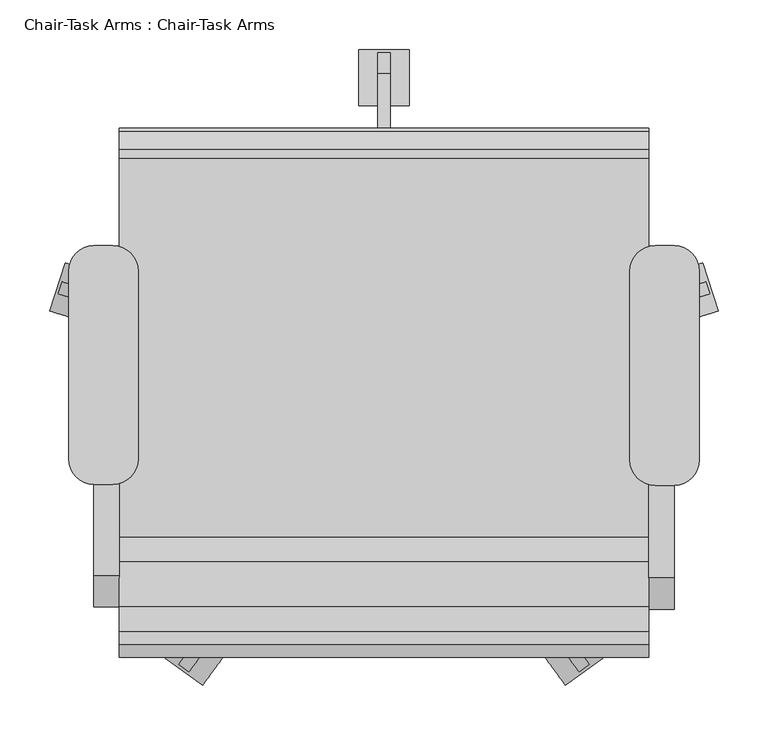
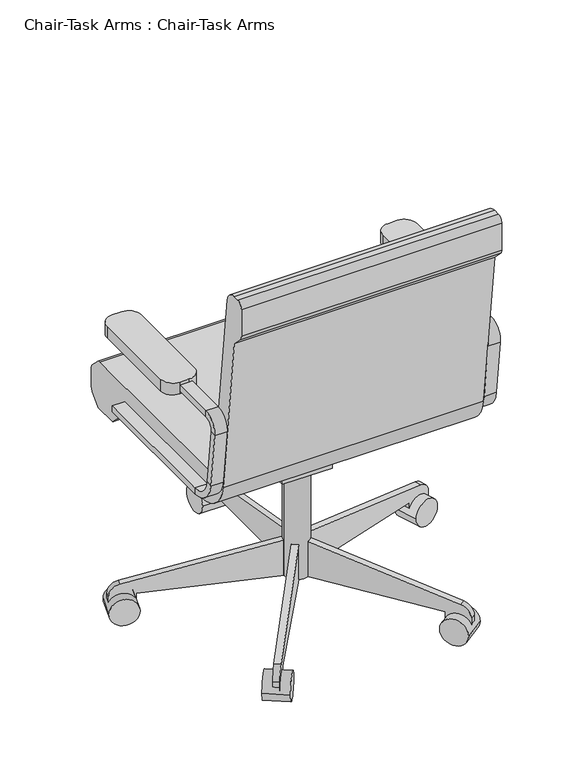
"""IFC4 building model written with IfcOpenShell, lengths in millimetres: furniture geometry, Chair-Task Arms : Chair-Task Arms."""

import ifcopenshell
import ifcopenshell.guid

model = None  # the IFC model being written
_history = None  # IfcOwnerHistory: only IFC2X3 demands one
_inside = {}  # id of a spatial element -> (the spatial element, [elements in it])
_under = {}  # id of a project, library or spatial element -> (it, [spatial elements below it])
_declared = {}  # id of a project -> (the project, [libraries it declares])
_typed = {}  # id of a type object -> (the type object, [elements of that type])
_made_of = {}  # id of a material, layer set ... -> (it, [elements and type objects made of it])


def new_model(schema):
    """Start an empty IFC model of exactly this schema.

    Asked for "IFC4X3", IfcOpenShell would pick the latest addendum, in which some entities
    have other attributes; the version numbers below select the first issue.
    IFC2X3 requires an IfcOwnerHistory on every rooted entity: one is made here for all.
    """
    global model, _history
    if schema == "IFC4X3":
        model = ifcopenshell.file(schema_version=(4, 3, 0, 0))
    else:
        model = ifcopenshell.file(schema=schema)
    _inside.clear()
    _under.clear()
    _declared.clear()
    _typed.clear()
    _made_of.clear()
    _history = None
    if model.schema == "IFC2X3":
        org = make("IfcOrganization", Name="unknown")
        user = make(
            "IfcPersonAndOrganization",
            ThePerson=make("IfcPerson", FamilyName="unknown"),
            TheOrganization=org,
        )
        app = make(
            "IfcApplication",
            ApplicationDeveloper=org,
            Version="unknown",
            ApplicationFullName="unknown",
            ApplicationIdentifier="unknown",
        )
        _history = make(
            "IfcOwnerHistory",
            OwningUser=user,
            OwningApplication=app,
            ChangeAction="ADDED",
            CreationDate=0,
        )
    return model


def make(cls, **values):
    """One entity of the class cls with the attributes given. An attribute that is None is left unset."""
    return model.create_entity(
        cls, **{name: value for name, value in values.items() if value is not None}
    )


def rooted(cls, **values):
    """An entity with a GlobalId (a new one), such as an element, a storey or a relation."""
    return make(cls, GlobalId=ifcopenshell.guid.new(), OwnerHistory=_history, **values)


def si_unit(unit_type, name, prefix=None):
    """IfcSIUnit, for example si_unit("LENGTHUNIT", "METRE", prefix="MILLI")."""
    return make("IfcSIUnit", UnitType=unit_type, Prefix=prefix, Name=name)


def assignment(units):
    """IfcUnitAssignment: the units of a project."""
    return None if units is None else make("IfcUnitAssignment", Units=units)


def point(xyz):
    """IfcCartesianPoint."""
    return None if xyz is None else make("IfcCartesianPoint", Coordinates=xyz)


def direction(xyz):
    """IfcDirection."""
    return None if xyz is None else make("IfcDirection", DirectionRatios=xyz)


def frame(location, z_axis=None, x_axis=None):
    """IfcAxis2Placement3D, a coordinate frame: its origin and axes. An axis left out is left unset."""
    return make(
        "IfcAxis2Placement3D",
        Location=point(location),
        Axis=direction(z_axis),
        RefDirection=direction(x_axis),
    )


def frame_2d(location, x_axis=None):
    """IfcAxis2Placement2D, a coordinate frame in the plane: its origin and x axis."""
    return make(
        "IfcAxis2Placement2D", Location=point(location), RefDirection=direction(x_axis)
    )


def origin():
    """The frame at (0, 0, 0) with its axes left unset."""
    return frame((0.0, 0.0, 0.0))


def place(relative_to, where):
    """IfcLocalPlacement: puts the frame where relative to a parent placement (None: the world)."""
    return make(
        "IfcLocalPlacement", PlacementRelTo=relative_to, RelativePlacement=where
    )


def context(
    kind, dimensions, precision=None, world=None, true_north=None, identifier=None
):
    """IfcGeometricRepresentationContext, for example the 3D "Model" context."""
    return make(
        "IfcGeometricRepresentationContext",
        ContextIdentifier=identifier,
        ContextType=kind,
        CoordinateSpaceDimension=dimensions,
        Precision=precision,
        WorldCoordinateSystem=world,
        TrueNorth=true_north,
    )


def project(units=None, contexts=None):
    """IfcProject with its units and contexts."""
    return rooted(
        "IfcProject",
        Name="project",
        RepresentationContexts=contexts,
        UnitsInContext=assignment(units),
    )


def spatial(cls, under=None, at=None, **own):
    """A site, building, storey or space (cls), placed at a placement, below another one or the project."""
    s = rooted(cls, ObjectPlacement=at, **own)
    if under is not None:
        _under.setdefault(under.id(), (under, []))[1].append(s)
    return s


def polyline(points):
    """IfcPolyline through the points."""
    return make("IfcPolyline", Points=[point(p) for p in points])


def circle_curve(where, radius):
    """IfcCircle in the frame where."""
    return make("IfcCircle", Position=where, Radius=radius)


def trimmed(basis, trim1, trim2, sense, master):
    """IfcTrimmedCurve: the piece of a basis curve between two trims."""
    return make(
        "IfcTrimmedCurve",
        BasisCurve=basis,
        Trim1=trim1,
        Trim2=trim2,
        SenseAgreement=sense,
        MasterRepresentation=master,
    )


def segment(curve, same_sense, transition):
    """IfcCompositeCurveSegment."""
    return make(
        "IfcCompositeCurveSegment",
        Transition=transition,
        SameSense=same_sense,
        ParentCurve=curve,
    )


def composite_curve(segments, self_intersect=None):
    """IfcCompositeCurve: segments joined end to end."""
    return make("IfcCompositeCurve", Segments=segments, SelfIntersect=self_intersect)


def outline(outer, holes=None, kind="AREA"):
    """IfcArbitraryClosedProfileDef: a profile drawn as a closed curve; with holes, ...WithVoids."""
    if holes is None:
        return make("IfcArbitraryClosedProfileDef", ProfileType=kind, OuterCurve=outer)
    return make(
        "IfcArbitraryProfileDefWithVoids",
        ProfileType=kind,
        OuterCurve=outer,
        InnerCurves=holes,
    )


def extrude(swept, where, along, depth):
    """IfcExtrudedAreaSolid: the profile swept, set in the frame where, extruded along a direction by depth."""
    return make(
        "IfcExtrudedAreaSolid",
        SweptArea=swept,
        Position=where,
        ExtrudedDirection=direction(along),
        Depth=depth,
    )


def shape(context_of_items, identifier, shape_type, items):
    """IfcShapeRepresentation: the items that make up one representation, for example the "Body"."""
    return make(
        "IfcShapeRepresentation",
        ContextOfItems=context_of_items,
        RepresentationIdentifier=identifier,
        RepresentationType=shape_type,
        Items=items,
    )


def source(mapping_origin, context_of_items, identifier, shape_type, items):
    """IfcRepresentationMap: a shape defined once, which mapped items show again and again."""
    return make(
        "IfcRepresentationMap",
        MappingOrigin=mapping_origin,
        MappedRepresentation=shape(context_of_items, identifier, shape_type, items),
    )


def transform(
    local_origin,
    x_axis=None,
    y_axis=None,
    z_axis=None,
    scale=None,
    scale2=None,
    scale3=None,
    uniform=True,
):
    """IfcCartesianTransformationOperator3D, or its non-uniform kind. x_axis, y_axis, z_axis: its Axis1, 2, 3."""
    if uniform:
        return make(
            "IfcCartesianTransformationOperator3D",
            Axis1=direction(x_axis),
            Axis2=direction(y_axis),
            LocalOrigin=point(local_origin),
            Scale=scale,
            Axis3=direction(z_axis),
        )
    return make(
        "IfcCartesianTransformationOperator3DnonUniform",
        Axis1=direction(x_axis),
        Axis2=direction(y_axis),
        LocalOrigin=point(local_origin),
        Scale=scale,
        Axis3=direction(z_axis),
        Scale2=scale2,
        Scale3=scale3,
    )


def mapped(mapping_source, mapping_target):
    """IfcMappedItem: shows the shape of a source again, moved by a transform."""
    return make(
        "IfcMappedItem", MappingSource=mapping_source, MappingTarget=mapping_target
    )


def made_of(thing, what):
    """Note that an element or type object is made of a material, layer set ...; save() writes the relation."""
    if what is not None:
        _made_of.setdefault(what.id(), (what, []))[1].append(thing)
    return thing


def element(
    cls,
    number,
    at=None,
    inside=None,
    cuts=None,
    type_object=None,
    material=None,
    context=None,
    identifier="Body",
    shape_type=None,
    held_by="IfcProductDefinitionShape",
    body=None,
    shapes=None,
    **own,
):
    """One element of the class cls, such as IfcWall. Its Tag is "e" and its number.

    at: its placement. inside: the storey or other place that contains it. cuts: it is an
    opening in that element (IfcRelVoidsElement). A single representation is given by context,
    identifier, shape_type and body (its items); several are given by shapes. held_by: the class
    of the entity that holds the representations. save() writes the other relations.
    """
    e = rooted(cls, Tag="e%d" % number, ObjectPlacement=at, **own)
    if body is not None:
        shapes = [shape(context, identifier, shape_type, body)]
    if shapes is not None:
        e.Representation = make(held_by, Representations=shapes)
    if inside is not None:
        _inside.setdefault(inside.id(), (inside, []))[1].append(e)
    if cuts is not None:
        rooted(
            "IfcRelVoidsElement", RelatingBuildingElement=cuts, RelatedOpeningElement=e
        )
    if type_object is not None:
        _typed.setdefault(type_object.id(), (type_object, []))[1].append(e)
    return made_of(e, material)


def aggregate(whole, parts):
    """IfcRelAggregates: a whole, such as a stair, and the parts it consists of."""
    return rooted("IfcRelAggregates", RelatingObject=whole, RelatedObjects=parts)


def save(model, path):
    """Write the relations noted so far, then the file.

    IfcRelAggregates (storeys below a building ...), IfcRelContainedInSpatialStructure (elements
    in a storey), IfcRelDefinesByType, IfcRelAssociatesMaterial and IfcRelDeclares: one each for
    every whole, place, type object, material and project.
    """
    for whole, parts in _under.values():
        aggregate(whole, parts)
    for where, things in _inside.values():
        rooted(
            "IfcRelContainedInSpatialStructure",
            RelatedElements=things,
            RelatingStructure=where,
        )
    for kind, things in _typed.values():
        rooted("IfcRelDefinesByType", RelatedObjects=things, RelatingType=kind)
    for what, things in _made_of.values():
        rooted("IfcRelAssociatesMaterial", RelatedObjects=things, RelatingMaterial=what)
    for by, libraries in _declared.values():
        rooted("IfcRelDeclares", RelatingContext=by, RelatedDefinitions=libraries)
    model.write(path)


def plane_surface(at):
    """IfcPlane: the flat surface through the origin of the frame at, square to its z axis."""
    return make("IfcPlane", Position=at)


def cylinder_surface(at, radius):
    """IfcCylindricalSurface: all points at the distance radius from the z axis of the frame at."""
    return make("IfcCylindricalSurface", Position=at, Radius=radius)


def revolved_surface(curve, axis_point, axis_direction):
    """IfcSurfaceOfRevolution: the curve turned about the line through axis_point along axis_direction."""
    return make(
        "IfcSurfaceOfRevolution",
        SweptCurve=make("IfcArbitraryOpenProfileDef", ProfileType="CURVE", Curve=curve),
        AxisPosition=make("IfcAxis1Placement", Location=point(axis_point), Axis=direction(axis_direction)),
    )


def advanced_brep(points, edges, surfaces, faces):
    """IfcAdvancedBrep: a solid bounded by faces that lie on surfaces and meet in shared edges.

    An edge is (start, end): straight between two places in points (the first is 0);
    or (start, end, curve); or (start, end, curve, False) where it runs against its curve.
    A face is (place in surfaces, loops), or (place, loops, False) where it looks against
    its surface's normal. A loop lists edges by number (the first is 1), with a minus sign
    where the edge is run from its end to its start. The first loop is the outer one.
    """
    corners = [point(p) for p in points]
    vertices = [make("IfcVertexPoint", VertexGeometry=c) for c in corners]
    made = []
    for start, end, *more in edges:
        made.append(
            make(
                "IfcEdgeCurve",
                EdgeStart=vertices[start],
                EdgeEnd=vertices[end],
                EdgeGeometry=more[0] if more else make("IfcPolyline", Points=[corners[start], corners[end]]),
                SameSense=more[1] if len(more) > 1 else True,
            )
        )
    hull = []
    for where, loops, *sense in faces:
        bounds = []
        for j, loop in enumerate(loops):
            ring = [make("IfcOrientedEdge", EdgeElement=made[abs(k) - 1], Orientation=k > 0) for k in loop]
            bounds.append(
                make(
                    "IfcFaceOuterBound" if j == 0 else "IfcFaceBound",
                    Bound=make("IfcEdgeLoop", EdgeList=ring),
                    Orientation=True,
                )
            )
        hull.append(make("IfcAdvancedFace", Bounds=bounds, FaceSurface=surfaces[where], SameSense=sense[0] if sense else True))
    return make("IfcAdvancedBrep", Outer=make("IfcClosedShell", CfsFaces=hull))


def chair_task_arms_chair_task_arms_fa5a08ef(model_context):
    return source(origin(), model_context, "Body", "SolidModel", [
        extrude(outline(composite_curve([segment(polyline([(433.0908197, -74.2028048), (414.0408197, -74.2028048)]), True, "CONTINUOUS"), segment(trimmed(circle_curve(frame_2d((414.0408197, -48.8028048)), 25.4), [point((414.0408197, -74.2028048))], [point((388.6408197, -48.8028048))], False, "CARTESIAN"), True, "CONTINUOUS"), segment(polyline([(388.6408197, -48.8028048), (388.6408197, 141.6319091)]), True, "CONTINUOUS"), segment(trimmed(circle_curve(frame_2d((414.0408197, 141.6319091)), 25.4), [point((388.6408197, 141.6319091))], [point((414.0408197, 167.0319091))], False, "CARTESIAN"), True, "CONTINUOUS"), segment(polyline([(414.0408197, 167.0319091), (433.0908197, 167.0319091)]), True, "CONTINUOUS"), segment(trimmed(circle_curve(frame_2d((433.0908197, 141.6319091)), 25.4), [point((433.0908197, 167.0319091))], [point((458.4908197, 141.6319091))], False, "CARTESIAN"), True, "CONTINUOUS"), segment(polyline([(458.4908197, 141.6319091), (458.4908197, -48.8028048)]), True, "CONTINUOUS"), segment(trimmed(circle_curve(frame_2d((433.0908197, -48.8028048)), 25.4), [point((458.4908197, -48.8028048))], [point((433.0908197, -74.2028048))], False, "CARTESIAN"), True, "CONTINUOUS")], self_intersect=False)), frame((0.0, 0.0, 596.9), z_axis=(0.0, 0.0, 1.0), x_axis=(1.0, 0.0, 0.0)), (0.0, 0.0, 1.0), 25.4),
        extrude(outline(composite_curve([segment(polyline([(-132.0591803, -73.1575984), (-151.1091803, -73.1575984)]), True, "CONTINUOUS"), segment(trimmed(circle_curve(frame_2d((-151.1091803, -47.7575984)), 25.4), [point((-151.1091803, -73.1575984))], [point((-176.5091803, -47.7575984))], False, "CARTESIAN"), True, "CONTINUOUS"), segment(polyline([(-176.5091803, -47.7575984), (-176.5091803, 141.6319091)]), True, "CONTINUOUS"), segment(trimmed(circle_curve(frame_2d((-151.1091803, 141.6319091)), 25.4), [point((-176.5091803, 141.6319091))], [point((-151.1091803, 167.0319091))], False, "CARTESIAN"), True, "CONTINUOUS"), segment(polyline([(-151.1091803, 167.0319091), (-132.0591803, 167.0319091)]), True, "CONTINUOUS"), segment(trimmed(circle_curve(frame_2d((-132.0591803, 141.6319091)), 25.4), [point((-132.0591803, 167.0319091))], [point((-106.6591803, 141.6319091))], False, "CARTESIAN"), True, "CONTINUOUS"), segment(polyline([(-106.6591803, 141.6319091), (-106.6591803, -47.7575984)]), True, "CONTINUOUS"), segment(trimmed(circle_curve(frame_2d((-132.0591803, -47.7575984)), 25.4), [point((-106.6591803, -47.7575984))], [point((-132.0591803, -73.1575984))], False, "CARTESIAN"), True, "CONTINUOUS")], self_intersect=False)), frame((0.0, 0.0, 596.9), z_axis=(0.0, 0.0, 1.0), x_axis=(1.0, 0.0, 0.0)), (0.0, 0.0, 1.0), 25.4),
        advanced_brep(
        [(-151.1091803, 167.0319091, 412.75), (-151.1091803, 167.0319091, 425.45), (-125.7091803, 167.0319091, 425.45), (-125.7091803, 167.0319091, 412.75), (-151.1091803, -126.2388651, 412.75), (-151.1091803, -126.2388651, 425.45), (-125.7091803, -126.2388651, 425.45), (-125.7091803, -126.2388651, 412.75), (-151.1091803, -170.3844094, 464.7064065), (-151.1091803, -182.9974221, 463.2225227), (-125.7091803, -170.3844094, 464.7064065), (-125.7091803, -182.9974221, 463.2225227), (-151.1091803, -196.7936301, 580.4902904), (-151.1091803, -184.1806174, 581.9741742), (-125.7091803, -184.1806174, 581.9741742), (-125.7091803, -196.7936301, 580.4902904), (-151.1091803, -165.2610984, 603.25), (-151.1091803, -165.2610984, 615.95), (-125.7091803, -165.2610984, 603.25), (-125.7091803, -165.2610984, 615.95), (-151.1091803, 18.9459016, 615.95), (-125.7091803, 18.9459016, 615.95), (-125.7091803, 18.9459016, 603.25), (-151.1091803, 18.9459016, 603.25)],
        [
            (0, 1),
            (1, 2),
            (2, 3),
            (3, 0),
            (0, 4),
            (4, 5),
            (5, 1),
            (5, 6),
            (6, 2),
            (6, 7),
            (7, 3),
            (7, 4),
            (8, 5, circle_curve(frame((-151.1091803, -126.2388651, 469.9), z_axis=(1.0, 0.0, 0.0), x_axis=(0.0, 0.0, -1.0)), 44.45)),
            (4, 9, circle_curve(frame((-151.1091803, -126.2388651, 469.9), z_axis=(-1.0, 0.0, 0.0), x_axis=(0.0, 0.0, -1.0)), 57.15)),
            (9, 8),
            (10, 6, circle_curve(frame((-125.7091803, -126.2388651, 469.9), z_axis=(1.0, 0.0, 0.0), x_axis=(0.0, 0.0, -1.0)), 44.45)),
            (8, 10),
            (11, 7, circle_curve(frame((-125.7091803, -126.2388651, 469.9), z_axis=(1.0, 0.0, 0.0), x_axis=(0.0, 0.0, -1.0)), 57.15)),
            (10, 11),
            (11, 9),
            (9, 12),
            (12, 13),
            (13, 8),
            (13, 14),
            (14, 10),
            (14, 15),
            (15, 11),
            (15, 12),
            (16, 13, circle_curve(frame((-151.1091803, -165.2610984, 584.2), z_axis=(1.0, 0.0, 0.0), x_axis=(0.0, -0.9931506043228768, -0.11684124756739202)), 19.05)),
            (12, 17, circle_curve(frame((-151.1091803, -165.2610984, 584.2), z_axis=(-1.0, 0.0, 0.0), x_axis=(0.0, -0.9931506043228768, -0.11684124756739202)), 31.75)),
            (17, 16),
            (18, 14, circle_curve(frame((-125.7091803, -165.2610984, 584.2), z_axis=(1.0, 0.0, 0.0), x_axis=(0.0, -0.9931506043228768, -0.11684124756739202)), 19.05)),
            (16, 18),
            (19, 15, circle_curve(frame((-125.7091803, -165.2610984, 584.2), z_axis=(1.0, 0.0, 0.0), x_axis=(0.0, -0.9931506043228768, -0.11684124756739202)), 31.75)),
            (18, 19),
            (19, 17),
            (20, 21),
            (21, 22),
            (22, 23),
            (23, 20),
            (17, 20),
            (23, 16),
            (22, 18),
            (21, 19),
        ],
        [
            plane_surface(frame((-152.608212, 167.0319091, 419.1), z_axis=(0.0, 1.0, 0.0), x_axis=(0.0, 0.0, -1.0))),
            plane_surface(frame((-151.1091803, 167.0319091, 412.75), z_axis=(-1.0, 0.0, 0.0), x_axis=(0.0, -1.0, 0.0))),
            plane_surface(frame((-151.1091803, 167.0319091, 425.45), z_axis=(0.0, 0.0, 1.0), x_axis=(0.0, -1.0, 0.0))),
            plane_surface(frame((-125.7091803, 167.0319091, 425.45), z_axis=(1.0, 0.0, 0.0), x_axis=(0.0, -1.0, 0.0))),
            plane_surface(frame((-125.7091803, 167.0319091, 412.75), z_axis=(0.0, 0.0, -1.0), x_axis=(0.0, -1.0, 0.0))),
            plane_surface(frame((-151.1091803, -126.2388651, 469.9), z_axis=(-1.0, 0.0, 0.0), x_axis=(0.0, 0.0, -1.0))),
            revolved_surface(polyline([(-151.1091803, -126.2388651, 425.45), (-125.7091803, -126.2388651, 425.45)]), (-138.4091803, -126.2388651, 469.9), (-1.0, 0.0, 0.0)),
            plane_surface(frame((-125.7091803, -126.2388651, 469.9), z_axis=(1.0, 0.0, 0.0), x_axis=(0.0, 0.0, -1.0))),
            cylinder_surface(frame((-138.4091803, -126.2388651, 469.9), z_axis=(-1.0, 0.0, 0.0), x_axis=(0.0, 0.0, -1.0)), 57.15),
            plane_surface(frame((-151.1091803, -182.9974221, 463.2225227), z_axis=(-1.0, 0.0, 0.0), x_axis=(0.0, -0.1168412475673856, 0.9931506043228776))),
            plane_surface(frame((-151.1091803, -170.3844094, 464.7064065), z_axis=(0.0, 0.9931506043228776, 0.1168412475673856), x_axis=(0.0, -0.1168412475673856, 0.9931506043228776))),
            plane_surface(frame((-125.7091803, -170.3844094, 464.7064065), z_axis=(1.0, 0.0, 0.0), x_axis=(0.0, -0.1168412475673856, 0.9931506043228776))),
            plane_surface(frame((-125.7091803, -182.9974221, 463.2225227), z_axis=(0.0, -0.9931506043228776, -0.1168412475673856), x_axis=(0.0, -0.1168412475673856, 0.9931506043228776))),
            plane_surface(frame((-151.1091803, -165.2610984, 584.2), z_axis=(-1.0, 0.0, 0.0), x_axis=(0.0, -0.9931506043228768, -0.11684124756739202))),
            revolved_surface(polyline([(-151.1091803, -184.1806174123508, 581.9741742338413), (-125.7091803, -184.1806174123508, 581.9741742338413)]), (-138.4091803, -165.2610984, 584.2), (-1.0, 0.0, 0.0)),
            plane_surface(frame((-125.7091803, -165.2610984, 584.2), z_axis=(1.0, 0.0, 0.0), x_axis=(0.0, -0.9931506043228768, -0.11684124756739202))),
            cylinder_surface(frame((-138.4091803, -165.2610984, 584.2), z_axis=(-1.0, 0.0, 0.0), x_axis=(0.0, -0.9931506043228768, -0.11684124756739202)), 31.75),
            plane_surface(frame((-152.608212, 18.9459016, 609.6), z_axis=(0.0, 1.0, 0.0), x_axis=(0.0, 0.0, 1.0))),
            plane_surface(frame((-151.1091803, -165.2610984, 615.95), z_axis=(-1.0, 0.0, 0.0), x_axis=(0.0, 1.0, 0.0))),
            plane_surface(frame((-151.1091803, -165.2610984, 603.25), z_axis=(0.0, 0.0, -1.0), x_axis=(0.0, 1.0, 0.0))),
            plane_surface(frame((-125.7091803, -165.2610984, 603.25), z_axis=(1.0, 0.0, 0.0), x_axis=(0.0, 1.0, 0.0))),
            plane_surface(frame((-125.7091803, -165.2610984, 615.95), z_axis=(0.0, 0.0, 1.0), x_axis=(0.0, 1.0, 0.0))),
        ],
        [
            (0, [[1, 2, 3, 4]]),
            (1, [[-1, 5, 6, 7]]),
            (2, [[-2, -7, 8, 9]]),
            (3, [[-3, -9, 10, 11]]),
            (4, [[-4, -11, 12, -5]]),
            (5, [[13, -6, 14, 15]]),
            (6, [[16, -8, -13, 17]]),
            (7, [[18, -10, -16, 19]]),
            (8, [[-14, -12, -18, 20]]),
            (9, [[-15, 21, 22, 23]]),
            (10, [[-17, -23, 24, 25]]),
            (11, [[-19, -25, 26, 27]]),
            (12, [[-20, -27, 28, -21]]),
            (13, [[29, -22, 30, 31]]),
            (14, [[32, -24, -29, 33]]),
            (15, [[34, -26, -32, 35]]),
            (16, [[-30, -28, -34, 36]]),
            (17, [[37, 38, 39, 40]]),
            (18, [[-31, 41, -40, 42]]),
            (19, [[-33, -42, -39, 43]]),
            (20, [[-35, -43, -38, 44]]),
            (21, [[-36, -44, -37, -41]]),
        ],
    ),
        advanced_brep(
        [(433.0908197, 167.0319091, 425.45), (433.0908197, 167.0319091, 412.75), (407.6908197, 167.0319091, 412.75), (407.6908197, 167.0319091, 425.45), (433.0908197, -128.329278, 425.45), (433.0908197, -128.329278, 412.75), (407.6908197, -128.329278, 412.75), (407.6908197, -128.329278, 425.45), (433.0908197, -185.0878351, 463.2225227), (433.0908197, -172.4748224, 464.7064065), (407.6908197, -185.0878351, 463.2225227), (407.6908197, -172.4748224, 464.7064065), (433.0908197, -186.2710303, 581.9741742), (433.0908197, -198.884043, 580.4902904), (407.6908197, -198.884043, 580.4902904), (407.6908197, -186.2710303, 581.9741742), (433.0908197, -167.3515113, 615.95), (433.0908197, -167.3515113, 603.25), (407.6908197, -167.3515113, 615.95), (407.6908197, -167.3515113, 603.25), (433.0908197, 18.9459016, 603.25), (407.6908197, 18.9459016, 603.25), (407.6908197, 18.9459016, 615.95), (433.0908197, 18.9459016, 615.95)],
        [
            (0, 1),
            (1, 2),
            (2, 3),
            (3, 0),
            (0, 4),
            (4, 5),
            (5, 1),
            (5, 6),
            (6, 2),
            (6, 7),
            (7, 3),
            (7, 4),
            (8, 5, circle_curve(frame((433.0908197, -128.329278, 469.9), z_axis=(1.0, 0.0, 0.0), x_axis=(0.0, 0.0, -1.0)), 57.15)),
            (4, 9, circle_curve(frame((433.0908197, -128.329278, 469.9), z_axis=(-1.0, 0.0, 0.0), x_axis=(0.0, 0.0, -1.0)), 44.45)),
            (9, 8),
            (10, 6, circle_curve(frame((407.6908197, -128.329278, 469.9), z_axis=(1.0, 0.0, 0.0), x_axis=(0.0, 0.0, -1.0)), 57.15)),
            (8, 10),
            (11, 7, circle_curve(frame((407.6908197, -128.329278, 469.9), z_axis=(1.0, 0.0, 0.0), x_axis=(0.0, 0.0, -1.0)), 44.45)),
            (10, 11),
            (11, 9),
            (9, 12),
            (12, 13),
            (13, 8),
            (13, 14),
            (14, 10),
            (14, 15),
            (15, 11),
            (15, 12),
            (16, 13, circle_curve(frame((433.0908197, -167.3515113, 584.2), z_axis=(1.0, 0.0, 0.0), x_axis=(0.0, -0.9931506043228767, -0.1168412475673929)), 31.75)),
            (12, 17, circle_curve(frame((433.0908197, -167.3515113, 584.2), z_axis=(-1.0, 0.0, 0.0), x_axis=(0.0, -0.9931506043228767, -0.1168412475673929)), 19.05)),
            (17, 16),
            (18, 14, circle_curve(frame((407.6908197, -167.3515113, 584.2), z_axis=(1.0, 0.0, 0.0), x_axis=(0.0, -0.9931506043228767, -0.1168412475673929)), 31.75)),
            (16, 18),
            (19, 15, circle_curve(frame((407.6908197, -167.3515113, 584.2), z_axis=(1.0, 0.0, 0.0), x_axis=(0.0, -0.9931506043228767, -0.1168412475673929)), 19.05)),
            (18, 19),
            (19, 17),
            (20, 21),
            (21, 22),
            (22, 23),
            (23, 20),
            (17, 20),
            (23, 16),
            (22, 18),
            (21, 19),
        ],
        [
            plane_surface(frame((406.191788, 167.0319091, 419.1), z_axis=(0.0, 1.0, 0.0), x_axis=(0.0, 0.0, -1.0))),
            plane_surface(frame((433.0908197, 167.0319091, 425.45), z_axis=(1.0, 0.0, 0.0), x_axis=(0.0, -1.0, 0.0))),
            plane_surface(frame((433.0908197, 167.0319091, 412.75), z_axis=(0.0, 0.0, -1.0), x_axis=(0.0, -1.0, 0.0))),
            plane_surface(frame((407.6908197, 167.0319091, 412.75), z_axis=(-1.0, 0.0, 0.0), x_axis=(0.0, -1.0, 0.0))),
            plane_surface(frame((407.6908197, 167.0319091, 425.45), z_axis=(0.0, 0.0, 1.0), x_axis=(0.0, -1.0, 0.0))),
            plane_surface(frame((433.0908197, -128.329278, 469.9), z_axis=(1.0, 0.0, 0.0), x_axis=(0.0, 0.0, -1.0))),
            cylinder_surface(frame((420.3908197, -128.329278, 469.9), z_axis=(-1.0, 0.0, 0.0), x_axis=(0.0, 0.0, -1.0)), 57.15),
            plane_surface(frame((407.6908197, -128.329278, 469.9), z_axis=(-1.0, 0.0, 0.0), x_axis=(0.0, 0.0, -1.0))),
            revolved_surface(polyline([(407.6908197, -128.329278, 425.45), (433.0908197, -128.329278, 425.45)]), (420.3908197, -128.329278, 469.9), (-1.0, 0.0, 0.0)),
            plane_surface(frame((433.0908197, -172.4748224, 464.7064065), z_axis=(1.0, 0.0, 0.0), x_axis=(0.0, -0.11684124756738626, 0.9931506043228775))),
            plane_surface(frame((433.0908197, -185.0878351, 463.2225227), z_axis=(0.0, -0.9931506043228775, -0.11684124756738655), x_axis=(0.0, -0.11684124756738655, 0.9931506043228775))),
            plane_surface(frame((407.6908197, -185.0878351, 463.2225227), z_axis=(-1.0, 0.0, 0.0), x_axis=(0.0, -0.11684124756738626, 0.9931506043228775))),
            plane_surface(frame((407.6908197, -172.4748224, 464.7064065), z_axis=(0.0, 0.9931506043228775, 0.11684124756738626), x_axis=(0.0, -0.11684124756738626, 0.9931506043228775))),
            plane_surface(frame((433.0908197, -167.3515113, 584.2), z_axis=(1.0, 0.0, 0.0), x_axis=(0.0, -0.9931506043228767, -0.1168412475673929))),
            cylinder_surface(frame((420.3908197, -167.3515113, 584.2), z_axis=(-1.0, 0.0, 0.0), x_axis=(0.0, -0.9931506043228767, -0.1168412475673929)), 31.75),
            plane_surface(frame((407.6908197, -167.3515113, 584.2), z_axis=(-1.0, 0.0, 0.0), x_axis=(0.0, -0.9931506043228767, -0.1168412475673929))),
            revolved_surface(polyline([(407.6908197, -186.2710303123508, 581.9741742338412), (433.0908197, -186.2710303123508, 581.9741742338412)]), (420.3908197, -167.3515113, 584.2), (-1.0, 0.0, 0.0)),
            plane_surface(frame((406.191788, 18.9459016, 609.6), z_axis=(0.0, 1.0, 0.0), x_axis=(0.0, 0.0, 1.0))),
            plane_surface(frame((433.0908197, -167.3515113, 603.25), z_axis=(1.0, 0.0, 0.0), x_axis=(0.0, 1.0, 0.0))),
            plane_surface(frame((433.0908197, -167.3515113, 615.95), z_axis=(0.0, 0.0, 1.0), x_axis=(0.0, 1.0, 0.0))),
            plane_surface(frame((407.6908197, -167.3515113, 615.95), z_axis=(-1.0, 0.0, 0.0), x_axis=(0.0, 1.0, 0.0))),
            plane_surface(frame((407.6908197, -167.3515113, 603.25), z_axis=(0.0, 0.0, -1.0), x_axis=(0.0, 1.0, 0.0))),
        ],
        [
            (0, [[1, 2, 3, 4]]),
            (1, [[-1, 5, 6, 7]]),
            (2, [[-2, -7, 8, 9]]),
            (3, [[-3, -9, 10, 11]]),
            (4, [[-4, -11, 12, -5]]),
            (5, [[13, -6, 14, 15]]),
            (6, [[16, -8, -13, 17]]),
            (7, [[18, -10, -16, 19]]),
            (8, [[-14, -12, -18, 20]]),
            (9, [[-15, 21, 22, 23]]),
            (10, [[-17, -23, 24, 25]]),
            (11, [[-19, -25, 26, 27]]),
            (12, [[-20, -27, 28, -21]]),
            (13, [[29, -22, 30, 31]]),
            (14, [[32, -24, -29, 33]]),
            (15, [[34, -26, -32, 35]]),
            (16, [[-30, -28, -34, 36]]),
            (17, [[37, 38, 39, 40]]),
            (18, [[-31, 41, -40, 42]]),
            (19, [[-33, -42, -39, 43]]),
            (20, [[-35, -43, -38, 44]]),
            (21, [[-36, -44, -37, -41]]),
        ],
    ),
        extrude(outline(composite_curve([segment(trimmed(circle_curve(frame_2d((140.9908197, 18.9459016)), 25.4), [point((115.5908197, 18.9459016))], [point((166.3908197, 18.9459016))], False, "CARTESIAN"), True, "CONTINUOUS"), segment(trimmed(circle_curve(frame_2d((140.9908197, 18.9459016)), 25.4), [point((166.3908197, 18.9459016))], [point((115.5908197, 18.9459016))], False, "CARTESIAN"), True, "CONTINUOUS")], self_intersect=False)), frame((0.0, 0.0, 53.5835944), z_axis=(0.0, 0.0, 1.0), x_axis=(1.0, 0.0, 0.0)), (0.0, 0.0, 1.0), 330.5914056),
        extrude(outline(composite_curve([segment(trimmed(circle_curve(frame_2d((0.0, -28.2002727)), 28.2002727), [point((0.0, -56.4005455))], [point((0.0, 0.0))], False, "CARTESIAN"), True, "CONTINUOUS"), segment(trimmed(circle_curve(frame_2d((0.0, -28.2002727)), 28.2002727), [point((0.0, 0.0))], [point((0.0, -56.4005455))], False, "CARTESIAN"), True, "CONTINUOUS")], self_intersect=False)), frame((477.6203484, 101.6163254, 28.1835944), z_axis=(-0.3090169943749423, 0.9510565162951553, 0.0), x_axis=(0.0, 0.0, 1.0)), (0.0, 0.0, 1.0), 50.8),
        extrude(outline(composite_curve([segment(polyline([(-25.4, 0.0), (0.0, 0.0), (0.0, -50.8), (-24.303053, -50.8)]), True, "CONTINUOUS"), segment(trimmed(circle_curve(frame_2d((-24.303053, -25.4)), 25.4), [point((-24.303053, -50.8))], [point((-49.3171699, -29.8106637))], False, "CARTESIAN"), True, "CONTINUOUS"), segment(polyline([(-49.3171699, -29.8106637), (-101.6, 266.7), (-101.6, 292.1), (-25.4, 292.1), (-25.4, 0.0)]), True, "CONTINUOUS")], self_intersect=False)), frame((420.756686, 103.1705568, 28.1835944), z_axis=(-0.3090169943749423, 0.9510565162951553, 0.0), x_axis=(0.0, 0.0, -1.0)), (0.0, 0.0, 1.0), 12.7),
        extrude(outline(composite_curve([segment(trimmed(circle_curve(frame_2d((0.0, -28.2002727)), 28.2002727), [point((0.0, -56.4005455))], [point((0.0, 0.0))], False, "CARTESIAN"), True, "CONTINUOUS"), segment(trimmed(circle_curve(frame_2d((0.0, -28.2002727)), 28.2002727), [point((0.0, 0.0))], [point((0.0, -56.4005455))], False, "CARTESIAN"), True, "CONTINUOUS")], self_intersect=False)), frame((323.63931, -275.6612394, 28.1835944), z_axis=(0.8090169943749499, 0.5877852522924699, 0.0), x_axis=(0.0, 0.0, 1.0)), (0.0, 0.0, 1.0), 50.8),
        extrude(outline(composite_curve([segment(polyline([(-25.4, 0.0), (0.0, 0.0), (0.0, -50.8), (-24.303053, -50.8)]), True, "CONTINUOUS"), segment(trimmed(circle_curve(frame_2d((-24.303053, -25.3999999)), 25.4), [point((-24.303053, -50.8))], [point((-49.3171699, -29.8106636))], False, "CARTESIAN"), True, "CONTINUOUS"), segment(polyline([(-49.3171699, -29.8106636), (-101.6, 266.7), (-101.6, 292.1), (-25.4, 292.1), (-25.4, 0.0)]), True, "CONTINUOUS")], self_intersect=False)), frame((307.545634, -221.1003988, 28.1835944), z_axis=(0.8090169943749499, 0.5877852522924699, 0.0), x_axis=(0.0, 0.0, -1.0)), (0.0, 0.0, 1.0), 12.7),
        extrude(outline(composite_curve([segment(trimmed(circle_curve(frame_2d((0.0, -28.2002727)), 28.2002727), [point((0.0, -56.4005455))], [point((0.0, 0.0))], False, "CARTESIAN"), True, "CONTINUOUS"), segment(trimmed(circle_curve(frame_2d((0.0, -28.2002727)), 28.2002727), [point((0.0, 0.0))], [point((0.0, -56.4005455))], False, "CARTESIAN"), True, "CONTINUOUS")], self_intersect=False)), frame((-41.6576707, -275.6612394, 28.1835944), z_axis=(-0.8090169943749458, 0.5877852522924754, 0.0), x_axis=(0.0, 0.0, -1.0)), (0.0, 0.0, 1.0), 50.8),
        extrude(outline(composite_curve([segment(polyline([(25.4, 0.0), (25.4, 292.1), (101.6, 292.1), (101.6, 266.7), (49.3171699, -29.8106637)]), True, "CONTINUOUS"), segment(trimmed(circle_curve(frame_2d((24.303053, -25.3999999)), 25.4), [point((49.3171699, -29.8106637))], [point((24.303053, -50.8))], False, "CARTESIAN"), True, "CONTINUOUS"), segment(polyline([(24.303053, -50.8), (0.0, -50.8), (0.0, 0.0), (25.4, 0.0)]), True, "CONTINUOUS")], self_intersect=False)), frame((-25.5639946, -221.1003988, 28.1835944), z_axis=(-0.8090169943749459, 0.5877852522924754, 0.0), x_axis=(0.0, 0.0, 1.0)), (0.0, 0.0, 1.0), 12.7),
        extrude(outline(composite_curve([segment(trimmed(circle_curve(frame_2d((0.0, -28.2002727)), 28.2002727), [point((0.0, -56.4005454))], [point((0.0, 0.0))], False, "CARTESIAN"), True, "CONTINUOUS"), segment(trimmed(circle_curve(frame_2d((0.0, -28.2002727)), 28.2002727), [point((0.0, 0.0))], [point((0.0, -56.4005454))], False, "CARTESIAN"), True, "CONTINUOUS")], self_intersect=False)), frame((-195.638709, 101.6163254, 28.1835944), z_axis=(0.3090169943749487, 0.9510565162951532, 0.0), x_axis=(0.0, 0.0, -1.0)), (0.0, 0.0, 1.0), 50.8),
        extrude(outline(composite_curve([segment(polyline([(25.4, 0.0), (25.4, 292.1000001), (101.6, 292.1000001), (101.6, 266.7), (49.3171699, -29.8106636)]), True, "CONTINUOUS"), segment(trimmed(circle_curve(frame_2d((24.303053, -25.4)), 25.4), [point((49.3171699, -29.8106636))], [point((24.303053, -50.8))], False, "CARTESIAN"), True, "CONTINUOUS"), segment(polyline([(24.303053, -50.8), (0.0, -50.8), (0.0, 0.0), (25.4, 0.0)]), True, "CONTINUOUS")], self_intersect=False)), frame((-138.7750467, 103.1705568, 28.1835944), z_axis=(0.3090169943749487, 0.9510565162951532, 0.0), x_axis=(0.0, 0.0, 1.0)), (0.0, 0.0, 1.0), 12.7),
        extrude(outline(composite_curve([segment(trimmed(circle_curve(frame_2d((336.4459016, 28.1835944)), 28.2002727), [point((308.2456289, 28.1835944))], [point((364.6461744, 28.1835944))], False, "CARTESIAN"), True, "CONTINUOUS"), segment(trimmed(circle_curve(frame_2d((336.4459016, 28.1835944)), 28.2002727), [point((364.6461744, 28.1835944))], [point((308.2456289, 28.1835944))], False, "CARTESIAN"), True, "CONTINUOUS")], self_intersect=False)), frame((115.5908197, 0.0, 0.0), z_axis=(1.0, 0.0, 0.0), x_axis=(0.0, 1.0, 0.0)), (0.0, 0.0, 1.0), 50.8),
        extrude(outline(composite_curve([segment(polyline([(311.0459016, 53.5835944), (18.9459016, 53.5835944), (18.9459016, 129.7835944), (44.3459016, 129.7835944), (340.8565654, 77.5007643)]), True, "CONTINUOUS"), segment(trimmed(circle_curve(frame_2d((336.4459016, 52.4866474)), 25.4), [point((340.8565654, 77.5007643))], [point((361.8459016, 52.4866474))], False, "CARTESIAN"), True, "CONTINUOUS"), segment(polyline([(361.8459016, 52.4866474), (361.8459016, 28.1835944), (311.0459016, 28.1835944), (311.0459016, 53.5835944)]), True, "CONTINUOUS")], self_intersect=False)), frame((134.6408197, 0.0, 0.0), z_axis=(1.0, 0.0, 0.0), x_axis=(0.0, 1.0, 0.0)), (0.0, 0.0, 1.0), 12.7),
        extrude(outline(polyline([(69.7459016, 383.7835944), (69.7459016, 371.0835944), (18.9459016, 283.0954134), (-19.1540984, 283.0954134), (-19.1540984, 383.7835944), (69.7459016, 383.7835944)])), frame((90.1908197, 0.0, 0.0), z_axis=(1.0, 0.0, 0.0), x_axis=(0.0, 1.0, 0.0)), (0.0, 0.0, 1.0), 101.6),
        extrude(outline(composite_curve([segment(polyline([(-126.2050455, 457.2), (255.0102301, 457.2)]), True, "CONTINUOUS"), segment(trimmed(circle_curve(frame_2d((255.0102301, 444.5)), 12.7), [point((255.0102301, 457.2))], [point((263.9604301, 453.510212))], False, "CARTESIAN"), True, "CONTINUOUS"), segment(polyline([(263.9604301, 453.510212), (281.8961016, 435.6939999)]), True, "CONTINUOUS"), segment(trimmed(circle_curve(frame_2d((272.9459016, 426.6837879)), 12.7), [point((281.8961016, 435.6939999))], [point((285.6459016, 426.6837879))], False, "CARTESIAN"), True, "CONTINUOUS"), segment(polyline([(285.6459016, 426.6837879), (285.6459016, 391.6405184)]), True, "CONTINUOUS"), segment(trimmed(circle_curve(frame_2d((260.2459016, 391.6405184)), 25.4), [point((285.6459016, 391.6405184))], [point((278.2663256, 373.7401184))], False, "CARTESIAN"), True, "CONTINUOUS"), segment(polyline([(278.2663256, 373.7401184), (260.2470284, 355.6), (209.4470284, 355.6), (181.0744602, 383.7835944), (-107.1089978, 383.7835944)]), True, "CONTINUOUS"), segment(trimmed(circle_curve(frame_2d((-107.1089978, 459.9835944)), 76.2), [point((-107.1089978, 383.7835944))], [point((-182.7870738, 451.0802913))], False, "CARTESIAN"), True, "CONTINUOUS"), segment(polyline([(-182.7870738, 451.0802913), (-222.3540984, 787.4), (-244.0343545, 809.0802561)]), True, "CONTINUOUS"), segment(trimmed(circle_curve(frame_2d((-235.0540984, 818.0605122)), 12.7), [point((-244.0343545, 809.0802561))], [point((-247.7540984, 818.0605122))], False, "CARTESIAN"), True, "CONTINUOUS"), segment(polyline([(-247.7540984, 818.0605122), (-247.7540984, 876.3)]), True, "CONTINUOUS"), segment(trimmed(circle_curve(frame_2d((-235.0540984, 876.3)), 12.7), [point((-247.7540984, 876.3))], [point((-235.0540984, 889.0))], False, "CARTESIAN"), True, "CONTINUOUS"), segment(polyline([(-235.0540984, 889.0), (-222.1789239, 889.0)]), True, "CONTINUOUS"), segment(trimmed(circle_curve(frame_2d((-222.1789239, 863.6)), 25.4), [point((-222.1789239, 889.0))], [point((-196.9528985, 866.5677677))], False, "CARTESIAN"), True, "CONTINUOUS"), segment(polyline([(-196.9528985, 866.5677677), (-151.4310708, 479.6322323)]), True, "CONTINUOUS"), segment(trimmed(circle_curve(frame_2d((-126.2050455, 482.6)), 25.4), [point((-151.4310708, 479.6322323))], [point((-126.2050455, 457.2))], True, "CARTESIAN"), True, "CONTINUOUS")], self_intersect=False)), frame((-125.7091803, 0.0, 0.0), z_axis=(1.0, 0.0, 0.0), x_axis=(0.0, 1.0, 0.0)), (0.0, 0.0, 1.0), 533.4),
    ])


if __name__ == "__main__":
    model = new_model("IFC4")
    model_context = context("Model", 3, world=origin())
    ifc_project = project(units=[si_unit("LENGTHUNIT", "METRE", prefix="MILLI")], contexts=[model_context])
    site = spatial("IfcSite", under=ifc_project)
    building = spatial("IfcBuilding", under=site)
    placement = place(None, origin())
    chair_task_arms_chair_task_arms_shape = chair_task_arms_chair_task_arms_fa5a08ef(model_context)
    element("IfcFurniture", 1, ObjectType="Chair-Task Arms : Chair-Task Arms", at=placement, inside=building, context=model_context, shape_type="MappedRepresentation", body=[
        mapped(chair_task_arms_chair_task_arms_shape, transform((0.0, 0.0, 0.0), x_axis=(1.0, 0.0, 0.0), y_axis=(0.0, 1.0, 0.0), z_axis=(0.0, 0.0, 1.0))),
    ])
    save(model, "model.ifc")

# Revit data of these elements
# Type "Chair-Task Arms : Chair-Task Arms"
#   Assembly Code = "E2020200"
#   Base Material = Plastic, Opaque Black
#   Caster Material = Plastic, Opaque Black
#   Seat/Back Material = Textile - Slate Blue
#   Default Elevation = 0
# Element 1 (IfcFurniture, "Chair-Task Arms : Chair-Task Arms")
#   Materials on its faces: "Plastic, Opaque Black", "Textile - Slate Blue"
# Materials
#   "Plastic, Opaque Black": class "Plastic", colour RGB 0 0 0, transparency 0, Description = "Plastic, generic, opaque black", Cost = 0
#   "Textile - Slate Blue": class "Fabric", colour RGB 98 102 118, transparency 0
